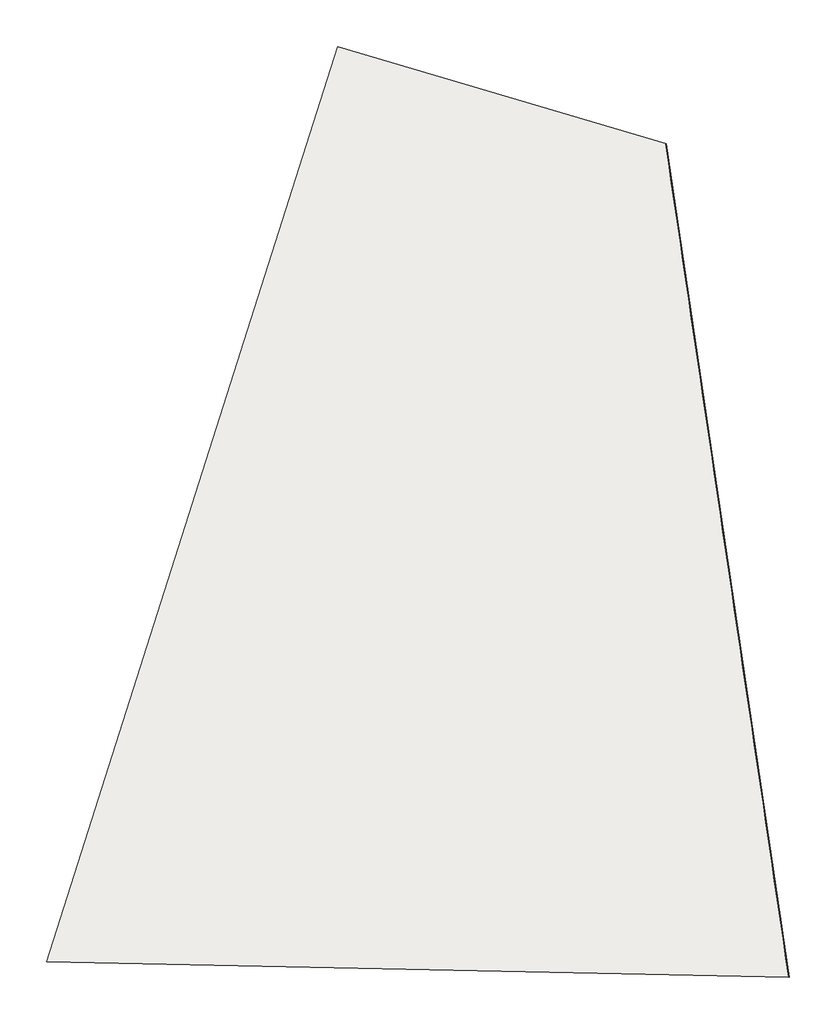
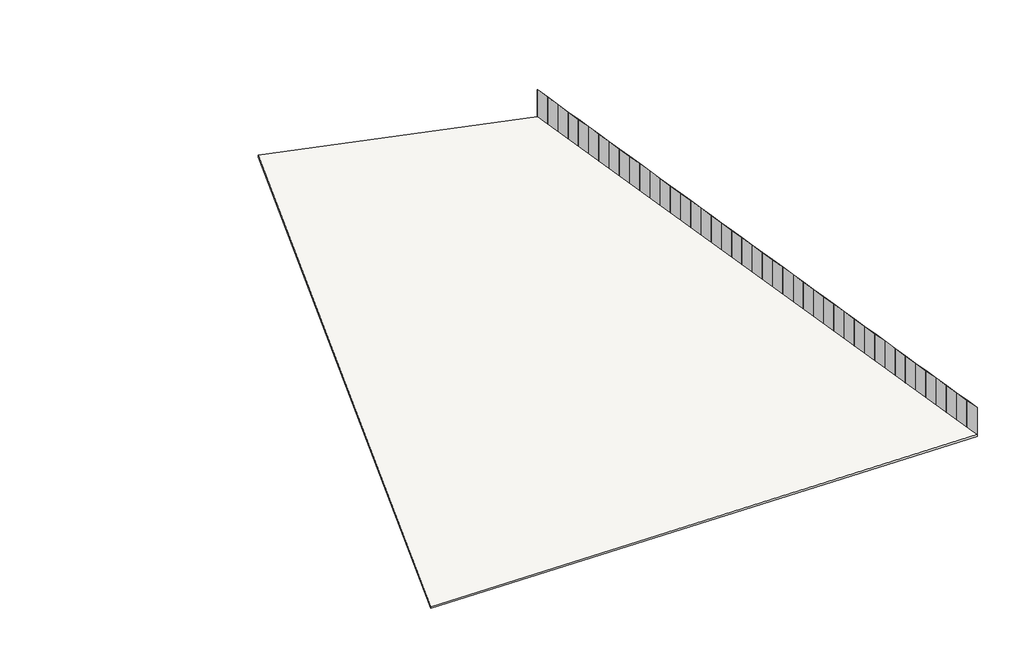
# One storey: 44 plates, 1 slab.
"""IFC4 building model written with IfcOpenShell, lengths in millimetres."""

import ifcopenshell
import ifcopenshell.guid

model = None  # the IFC model being written
_history = None  # IfcOwnerHistory: only IFC2X3 demands one
_inside = {}  # id of a spatial element -> (the spatial element, [elements in it])
_under = {}  # id of a project, library or spatial element -> (it, [spatial elements below it])
_declared = {}  # id of a project -> (the project, [libraries it declares])
_typed = {}  # id of a type object -> (the type object, [elements of that type])
_made_of = {}  # id of a material, layer set ... -> (it, [elements and type objects made of it])


def new_model(schema):
    """Start an empty IFC model of exactly this schema.

    Asked for "IFC4X3", IfcOpenShell would pick the latest addendum, in which some entities
    have other attributes; the version numbers below select the first issue.
    IFC2X3 requires an IfcOwnerHistory on every rooted entity: one is made here for all.
    """
    global model, _history
    if schema == "IFC4X3":
        model = ifcopenshell.file(schema_version=(4, 3, 0, 0))
    else:
        model = ifcopenshell.file(schema=schema)
    _inside.clear()
    _under.clear()
    _declared.clear()
    _typed.clear()
    _made_of.clear()
    _history = None
    if model.schema == "IFC2X3":
        org = make("IfcOrganization", Name="unknown")
        user = make(
            "IfcPersonAndOrganization",
            ThePerson=make("IfcPerson", FamilyName="unknown"),
            TheOrganization=org,
        )
        app = make(
            "IfcApplication",
            ApplicationDeveloper=org,
            Version="unknown",
            ApplicationFullName="unknown",
            ApplicationIdentifier="unknown",
        )
        _history = make(
            "IfcOwnerHistory",
            OwningUser=user,
            OwningApplication=app,
            ChangeAction="ADDED",
            CreationDate=0,
        )
    return model


def make(cls, **values):
    """One entity of the class cls with the attributes given. An attribute that is None is left unset."""
    return model.create_entity(
        cls, **{name: value for name, value in values.items() if value is not None}
    )


def rooted(cls, **values):
    """An entity with a GlobalId (a new one), such as an element, a storey or a relation."""
    return make(cls, GlobalId=ifcopenshell.guid.new(), OwnerHistory=_history, **values)


def si_unit(unit_type, name, prefix=None):
    """IfcSIUnit, for example si_unit("LENGTHUNIT", "METRE", prefix="MILLI")."""
    return make("IfcSIUnit", UnitType=unit_type, Prefix=prefix, Name=name)


def assignment(units):
    """IfcUnitAssignment: the units of a project."""
    return None if units is None else make("IfcUnitAssignment", Units=units)


def point(xyz):
    """IfcCartesianPoint."""
    return None if xyz is None else make("IfcCartesianPoint", Coordinates=xyz)


def direction(xyz):
    """IfcDirection."""
    return None if xyz is None else make("IfcDirection", DirectionRatios=xyz)


def frame(location, z_axis=None, x_axis=None):
    """IfcAxis2Placement3D, a coordinate frame: its origin and axes. An axis left out is left unset."""
    return make(
        "IfcAxis2Placement3D",
        Location=point(location),
        Axis=direction(z_axis),
        RefDirection=direction(x_axis),
    )


def origin():
    """The frame at (0, 0, 0) with its axes left unset."""
    return frame((0.0, 0.0, 0.0))


def origin_with_axes():
    """The frame at (0, 0, 0) with the z axis (0, 0, 1) and the x axis (1, 0, 0) written out."""
    return frame((0.0, 0.0, 0.0), z_axis=(0.0, 0.0, 1.0), x_axis=(1.0, 0.0, 0.0))


def place(relative_to, where):
    """IfcLocalPlacement: puts the frame where relative to a parent placement (None: the world)."""
    return make(
        "IfcLocalPlacement", PlacementRelTo=relative_to, RelativePlacement=where
    )


def context(
    kind, dimensions, precision=None, world=None, true_north=None, identifier=None
):
    """IfcGeometricRepresentationContext, for example the 3D "Model" context."""
    return make(
        "IfcGeometricRepresentationContext",
        ContextIdentifier=identifier,
        ContextType=kind,
        CoordinateSpaceDimension=dimensions,
        Precision=precision,
        WorldCoordinateSystem=world,
        TrueNorth=true_north,
    )


def project(units=None, contexts=None):
    """IfcProject with its units and contexts."""
    return rooted(
        "IfcProject",
        Name="project",
        RepresentationContexts=contexts,
        UnitsInContext=assignment(units),
    )


def spatial(cls, under=None, at=None, **own):
    """A site, building, storey or space (cls), placed at a placement, below another one or the project."""
    s = rooted(cls, ObjectPlacement=at, **own)
    if under is not None:
        _under.setdefault(under.id(), (under, []))[1].append(s)
    return s


def polyline(points):
    """IfcPolyline through the points."""
    return make("IfcPolyline", Points=[point(p) for p in points])


def outline(outer, holes=None, kind="AREA"):
    """IfcArbitraryClosedProfileDef: a profile drawn as a closed curve; with holes, ...WithVoids."""
    if holes is None:
        return make("IfcArbitraryClosedProfileDef", ProfileType=kind, OuterCurve=outer)
    return make(
        "IfcArbitraryProfileDefWithVoids",
        ProfileType=kind,
        OuterCurve=outer,
        InnerCurves=holes,
    )


def extrude(swept, where, along, depth):
    """IfcExtrudedAreaSolid: the profile swept, set in the frame where, extruded along a direction by depth."""
    return make(
        "IfcExtrudedAreaSolid",
        SweptArea=swept,
        Position=where,
        ExtrudedDirection=direction(along),
        Depth=depth,
    )


def shape(context_of_items, identifier, shape_type, items):
    """IfcShapeRepresentation: the items that make up one representation, for example the "Body"."""
    return make(
        "IfcShapeRepresentation",
        ContextOfItems=context_of_items,
        RepresentationIdentifier=identifier,
        RepresentationType=shape_type,
        Items=items,
    )


def source(mapping_origin, context_of_items, identifier, shape_type, items):
    """IfcRepresentationMap: a shape defined once, which mapped items show again and again."""
    return make(
        "IfcRepresentationMap",
        MappingOrigin=mapping_origin,
        MappedRepresentation=shape(context_of_items, identifier, shape_type, items),
    )


def transform(
    local_origin,
    x_axis=None,
    y_axis=None,
    z_axis=None,
    scale=None,
    scale2=None,
    scale3=None,
    uniform=True,
):
    """IfcCartesianTransformationOperator3D, or its non-uniform kind. x_axis, y_axis, z_axis: its Axis1, 2, 3."""
    if uniform:
        return make(
            "IfcCartesianTransformationOperator3D",
            Axis1=direction(x_axis),
            Axis2=direction(y_axis),
            LocalOrigin=point(local_origin),
            Scale=scale,
            Axis3=direction(z_axis),
        )
    return make(
        "IfcCartesianTransformationOperator3DnonUniform",
        Axis1=direction(x_axis),
        Axis2=direction(y_axis),
        LocalOrigin=point(local_origin),
        Scale=scale,
        Axis3=direction(z_axis),
        Scale2=scale2,
        Scale3=scale3,
    )


def mapped(mapping_source, mapping_target):
    """IfcMappedItem: shows the shape of a source again, moved by a transform."""
    return make(
        "IfcMappedItem", MappingSource=mapping_source, MappingTarget=mapping_target
    )


def made_of(thing, what):
    """Note that an element or type object is made of a material, layer set ...; save() writes the relation."""
    if what is not None:
        _made_of.setdefault(what.id(), (what, []))[1].append(thing)
    return thing


def element(
    cls,
    number,
    at=None,
    inside=None,
    cuts=None,
    type_object=None,
    material=None,
    context=None,
    identifier="Body",
    shape_type=None,
    held_by="IfcProductDefinitionShape",
    body=None,
    shapes=None,
    **own,
):
    """One element of the class cls, such as IfcWall. Its Tag is "e" and its number.

    at: its placement. inside: the storey or other place that contains it. cuts: it is an
    opening in that element (IfcRelVoidsElement). A single representation is given by context,
    identifier, shape_type and body (its items); several are given by shapes. held_by: the class
    of the entity that holds the representations. save() writes the other relations.
    """
    e = rooted(cls, Tag="e%d" % number, ObjectPlacement=at, **own)
    if body is not None:
        shapes = [shape(context, identifier, shape_type, body)]
    if shapes is not None:
        e.Representation = make(held_by, Representations=shapes)
    if inside is not None:
        _inside.setdefault(inside.id(), (inside, []))[1].append(e)
    if cuts is not None:
        rooted(
            "IfcRelVoidsElement", RelatingBuildingElement=cuts, RelatedOpeningElement=e
        )
    if type_object is not None:
        _typed.setdefault(type_object.id(), (type_object, []))[1].append(e)
    return made_of(e, material)


def aggregate(whole, parts):
    """IfcRelAggregates: a whole, such as a stair, and the parts it consists of."""
    return rooted("IfcRelAggregates", RelatingObject=whole, RelatedObjects=parts)


def save(model, path):
    """Write the relations noted so far, then the file.

    IfcRelAggregates (storeys below a building ...), IfcRelContainedInSpatialStructure (elements
    in a storey), IfcRelDefinesByType, IfcRelAssociatesMaterial and IfcRelDeclares: one each for
    every whole, place, type object, material and project.
    """
    for whole, parts in _under.values():
        aggregate(whole, parts)
    for where, things in _inside.values():
        rooted(
            "IfcRelContainedInSpatialStructure",
            RelatedElements=things,
            RelatingStructure=where,
        )
    for kind, things in _typed.values():
        rooted("IfcRelDefinesByType", RelatedObjects=things, RelatingType=kind)
    for what, things in _made_of.values():
        rooted("IfcRelAssociatesMaterial", RelatedObjects=things, RelatingMaterial=what)
    for by, libraries in _declared.values():
        rooted("IfcRelDeclares", RelatingContext=by, RelatedDefinitions=libraries)
    model.write(path)


def painel_do_sistema_1cdad03e(model_context):
    return source(origin(), model_context, "Body", "SweptSolid", [
        extrude(outline(polyline([(1500.0, 24.5), (-1500.0, 24.5), (-1500.0, 49.5), (1500.0, 49.5), (1500.0, 24.5)])), origin_with_axes(), (0.0, 0.0, 1.0), 1500.0),
    ])


def painel_do_sistema_6129cf31(model_context):
    return source(origin(), model_context, "Body", "SweptSolid", [
        extrude(outline(polyline([(0.0, -1500.0), (0.0, -332.3130513), (0.0, 1500.0), (20.0931032, 1500.0), (20.0931032, -1500.0), (0.0, -1500.0)])), frame((0.0, 24.5, 0.0), z_axis=(0.0, 1.0, 0.0), x_axis=(0.0, 0.0, 1.0)), (0.0, 0.0, 1.0), 25.0),
    ])


model = new_model("IFC4")

# Units and contexts
model_context = context("Model", 3, world=origin())
ifc_project = project(units=[si_unit("LENGTHUNIT", "METRE", prefix="MILLI")], contexts=[model_context])

# Site, building, storey
site = spatial("IfcSite", under=ifc_project)
building = spatial("IfcBuilding", under=site)
storey = spatial("IfcBuildingStorey", under=building, Name="Nível 2", Elevation=3000.0)

# Plates
placement = place(None, origin())
painel_do_sistema_shape = painel_do_sistema_1cdad03e(model_context)
element("IfcPlate", 1, ObjectType="Painel do sistema : Envidraçado", at=placement, inside=storey, context=model_context, shape_type="MappedRepresentation", body=[
    mapped(painel_do_sistema_shape, transform((27835.0106579, -36774.1442579, 4500.000015), x_axis=(0.0, 0.0, 1.0), y_axis=(-0.9892699032546328, -0.1460994815684493, 0.0), z_axis=(0.1460994815684493, -0.9892699032546328, 0.0))),
])
element("IfcPlate", 2, ObjectType="Painel do sistema : Envidraçado", at=placement, inside=storey, context=model_context, shape_type="MappedRepresentation", body=[
    mapped(painel_do_sistema_shape, transform((27615.8614356, -35290.239403, 4500.000015), x_axis=(0.0, 0.0, 1.0), y_axis=(-0.9892699032546328, -0.14609948156844887, 0.0), z_axis=(0.14609948156844887, -0.9892699032546328, 0.0))),
])
element("IfcPlate", 3, ObjectType="Painel do sistema : Envidraçado", at=placement, inside=storey, context=model_context, shape_type="MappedRepresentation", body=[
    mapped(painel_do_sistema_shape, transform((27396.7122132, -33806.3345481, 4500.000015), x_axis=(0.0, 0.0, 1.0), y_axis=(-0.9892699032546323, -0.1460994815684521, 0.0), z_axis=(0.1460994815684521, -0.9892699032546323, 0.0))),
])
element("IfcPlate", 4, ObjectType="Painel do sistema : Envidraçado", at=placement, inside=storey, context=model_context, shape_type="MappedRepresentation", body=[
    mapped(painel_do_sistema_shape, transform((27177.5629909, -32322.4296932, 4500.000015), x_axis=(0.0, 0.0, 1.0), y_axis=(-0.9892699032546327, -0.14609948156844926, 0.0), z_axis=(0.14609948156844926, -0.9892699032546327, 0.0))),
])
element("IfcPlate", 5, ObjectType="Painel do sistema : Envidraçado", at=placement, inside=storey, context=model_context, shape_type="MappedRepresentation", body=[
    mapped(painel_do_sistema_shape, transform((26958.4137685, -30838.5248383, 4500.000015), x_axis=(0.0, 0.0, 1.0), y_axis=(-0.9892699032546327, -0.1460994815684493, 0.0), z_axis=(0.1460994815684493, -0.9892699032546327, 0.0))),
])
element("IfcPlate", 6, ObjectType="Painel do sistema : Envidraçado", at=placement, inside=storey, context=model_context, shape_type="MappedRepresentation", body=[
    mapped(painel_do_sistema_shape, transform((26739.2645462, -29354.6199835, 4500.000015), x_axis=(0.0, 0.0, 1.0), y_axis=(-0.9892699032546327, -0.1460994815684493, 0.0), z_axis=(0.1460994815684493, -0.9892699032546327, 0.0))),
])
element("IfcPlate", 7, ObjectType="Painel do sistema : Envidraçado", at=placement, inside=storey, context=model_context, shape_type="MappedRepresentation", body=[
    mapped(painel_do_sistema_shape, transform((26520.1153238, -27870.7151286, 4500.000015), x_axis=(0.0, 0.0, 1.0), y_axis=(-0.9892699032546324, -0.1460994815684517, 0.0), z_axis=(0.1460994815684517, -0.9892699032546324, 0.0))),
])
element("IfcPlate", 8, ObjectType="Painel do sistema : Envidraçado", at=placement, inside=storey, context=model_context, shape_type="MappedRepresentation", body=[
    mapped(painel_do_sistema_shape, transform((26300.9661014, -26386.8102737, 4500.000015), x_axis=(0.0, 0.0, 1.0), y_axis=(-0.9892699032546328, -0.1460994815684493, 0.0), z_axis=(0.1460994815684493, -0.9892699032546328, 0.0))),
])
element("IfcPlate", 9, ObjectType="Painel do sistema : Envidraçado", at=placement, inside=storey, context=model_context, shape_type="MappedRepresentation", body=[
    mapped(painel_do_sistema_shape, transform((26081.8168791, -24902.9054188, 4500.000015), x_axis=(0.0, 0.0, 1.0), y_axis=(-0.9892699032546328, -0.14609948156844887, 0.0), z_axis=(0.14609948156844887, -0.9892699032546328, 0.0))),
])
element("IfcPlate", 10, ObjectType="Painel do sistema : Envidraçado", at=placement, inside=storey, context=model_context, shape_type="MappedRepresentation", body=[
    mapped(painel_do_sistema_shape, transform((25862.6676567, -23419.0005639, 4500.000015), x_axis=(0.0, 0.0, 1.0), y_axis=(-0.9892699032546324, -0.1460994815684517, 0.0), z_axis=(0.1460994815684517, -0.9892699032546324, 0.0))),
])
element("IfcPlate", 11, ObjectType="Painel do sistema : Envidraçado", at=placement, inside=storey, context=model_context, shape_type="MappedRepresentation", body=[
    mapped(painel_do_sistema_shape, transform((25643.5184344, -21935.095709, 4500.000015), x_axis=(0.0, 0.0, 1.0), y_axis=(-0.9892699032546328, -0.1460994815684493, 0.0), z_axis=(0.1460994815684493, -0.9892699032546328, 0.0))),
])
element("IfcPlate", 12, ObjectType="Painel do sistema : Envidraçado", at=placement, inside=storey, context=model_context, shape_type="MappedRepresentation", body=[
    mapped(painel_do_sistema_shape, transform((25424.369212, -20451.1908542, 4500.000015), x_axis=(0.0, 0.0, 1.0), y_axis=(-0.9892699032546324, -0.1460994815684517, 0.0), z_axis=(0.1460994815684517, -0.9892699032546324, 0.0))),
])
element("IfcPlate", 13, ObjectType="Painel do sistema : Envidraçado", at=placement, inside=storey, context=model_context, shape_type="MappedRepresentation", body=[
    mapped(painel_do_sistema_shape, transform((25205.2199897, -18967.2859993, 4500.000015), x_axis=(0.0, 0.0, 1.0), y_axis=(-0.9892699032546328, -0.14609948156844868, 0.0), z_axis=(0.14609948156844868, -0.9892699032546328, 0.0))),
])
element("IfcPlate", 14, ObjectType="Painel do sistema : Envidraçado", at=placement, inside=storey, context=model_context, shape_type="MappedRepresentation", body=[
    mapped(painel_do_sistema_shape, transform((24986.0707673, -17483.3811444, 4500.000015), x_axis=(0.0, 0.0, 1.0), y_axis=(-0.9892699032546328, -0.1460994815684491, 0.0), z_axis=(0.1460994815684491, -0.9892699032546328, 0.0))),
])
element("IfcPlate", 15, ObjectType="Painel do sistema : Envidraçado", at=placement, inside=storey, context=model_context, shape_type="MappedRepresentation", body=[
    mapped(painel_do_sistema_shape, transform((24766.921545, -15999.4762895, 4500.000015), x_axis=(0.0, 0.0, 1.0), y_axis=(-0.9892699032546328, -0.1460994815684493, 0.0), z_axis=(0.1460994815684493, -0.9892699032546328, 0.0))),
])
element("IfcPlate", 16, ObjectType="Painel do sistema : Envidraçado", at=placement, inside=storey, context=model_context, shape_type="MappedRepresentation", body=[
    mapped(painel_do_sistema_shape, transform((24547.7723226, -14515.5714346, 4500.000015), x_axis=(0.0, 0.0, 1.0), y_axis=(-0.9892699032546324, -0.1460994815684517, 0.0), z_axis=(0.1460994815684517, -0.9892699032546324, 0.0))),
])
element("IfcPlate", 17, ObjectType="Painel do sistema : Envidraçado", at=placement, inside=storey, context=model_context, shape_type="MappedRepresentation", body=[
    mapped(painel_do_sistema_shape, transform((24328.6231003, -13031.6665798, 4500.000015), x_axis=(0.0, 0.0, 1.0), y_axis=(-0.9892699032546327, -0.1460994815684495, 0.0), z_axis=(0.1460994815684495, -0.9892699032546327, 0.0))),
])
element("IfcPlate", 18, ObjectType="Painel do sistema : Envidraçado", at=placement, inside=storey, context=model_context, shape_type="MappedRepresentation", body=[
    mapped(painel_do_sistema_shape, transform((24109.4738779, -11547.7617249, 4500.000015), x_axis=(0.0, 0.0, 1.0), y_axis=(-0.9892699032546328, -0.1460994815684491, 0.0), z_axis=(0.1460994815684491, -0.9892699032546328, 0.0))),
])
element("IfcPlate", 19, ObjectType="Painel do sistema : Envidraçado", at=placement, inside=storey, context=model_context, shape_type="MappedRepresentation", body=[
    mapped(painel_do_sistema_shape, transform((23890.3246556, -10063.85687, 4500.000015), x_axis=(0.0, 0.0, 1.0), y_axis=(-0.9892699032546324, -0.14609948156845148, 0.0), z_axis=(0.14609948156845148, -0.9892699032546324, 0.0))),
])
element("IfcPlate", 20, ObjectType="Painel do sistema : Envidraçado", at=placement, inside=storey, context=model_context, shape_type="MappedRepresentation", body=[
    mapped(painel_do_sistema_shape, transform((23671.1754332, -8579.9520151, 4500.000015), x_axis=(0.0, 0.0, 1.0), y_axis=(-0.9892699032546332, -0.14609948156844624, 0.0), z_axis=(0.14609948156844624, -0.9892699032546332, 0.0))),
])
element("IfcPlate", 21, ObjectType="Painel do sistema : Envidraçado", at=placement, inside=storey, context=model_context, shape_type="MappedRepresentation", body=[
    mapped(painel_do_sistema_shape, transform((23452.0262109, -7096.0471602, 4500.000015), x_axis=(0.0, 0.0, 1.0), y_axis=(-0.9892699032546319, -0.14609948156845473, 0.0), z_axis=(0.14609948156845473, -0.9892699032546319, 0.0))),
])
element("IfcPlate", 22, ObjectType="Painel do sistema : Envidraçado", at=placement, inside=storey, context=model_context, shape_type="MappedRepresentation", body=[
    mapped(painel_do_sistema_shape, transform((23232.8769885, -5612.1423053, 4500.000015), x_axis=(0.0, 0.0, 1.0), y_axis=(-0.9892699032546332, -0.14609948156844646, 0.0), z_axis=(0.14609948156844646, -0.9892699032546332, 0.0))),
])
element("IfcPlate", 23, ObjectType="Painel do sistema : Envidraçado", at=placement, inside=storey, context=model_context, shape_type="MappedRepresentation", body=[
    mapped(painel_do_sistema_shape, transform((23013.7277662, -4128.2374505, 4500.000015), x_axis=(0.0, 0.0, 1.0), y_axis=(-0.9892699032546324, -0.1460994815684517, 0.0), z_axis=(0.1460994815684517, -0.9892699032546324, 0.0))),
])
element("IfcPlate", 24, ObjectType="Painel do sistema : Envidraçado", at=placement, inside=storey, context=model_context, shape_type="MappedRepresentation", body=[
    mapped(painel_do_sistema_shape, transform((22794.5785438, -2644.3325956, 4500.000015), x_axis=(0.0, 0.0, 1.0), y_axis=(-0.9892699032546328, -0.14609948156844865, 0.0), z_axis=(0.14609948156844865, -0.9892699032546328, 0.0))),
])
element("IfcPlate", 25, ObjectType="Painel do sistema : Envidraçado", at=placement, inside=storey, context=model_context, shape_type="MappedRepresentation", body=[
    mapped(painel_do_sistema_shape, transform((22575.4293215, -1160.4277407, 4500.000015), x_axis=(0.0, 0.0, 1.0), y_axis=(-0.9892699032546327, -0.1460994815684493, 0.0), z_axis=(0.1460994815684493, -0.9892699032546327, 0.0))),
])
element("IfcPlate", 26, ObjectType="Painel do sistema : Envidraçado", at=placement, inside=storey, context=model_context, shape_type="MappedRepresentation", body=[
    mapped(painel_do_sistema_shape, transform((22356.2800991, 323.4771142, 4500.000015), x_axis=(0.0, 0.0, 1.0), y_axis=(-0.9892699032546324, -0.14609948156845148, 0.0), z_axis=(0.14609948156845148, -0.9892699032546324, 0.0))),
])
element("IfcPlate", 27, ObjectType="Painel do sistema : Envidraçado", at=placement, inside=storey, context=model_context, shape_type="MappedRepresentation", body=[
    mapped(painel_do_sistema_shape, transform((22137.1308767, 1807.3819691, 4500.000015), x_axis=(0.0, 0.0, 1.0), y_axis=(-0.9892699032546332, -0.1460994815684469, 0.0), z_axis=(0.1460994815684469, -0.9892699032546332, 0.0))),
])
element("IfcPlate", 28, ObjectType="Painel do sistema : Envidraçado", at=placement, inside=storey, context=model_context, shape_type="MappedRepresentation", body=[
    mapped(painel_do_sistema_shape, transform((21917.9816544, 3291.2868239, 4500.000015), x_axis=(0.0, 0.0, 1.0), y_axis=(-0.9892699032546323, -0.1460994815684521, 0.0), z_axis=(0.1460994815684521, -0.9892699032546323, 0.0))),
])
element("IfcPlate", 29, ObjectType="Painel do sistema : Envidraçado", at=placement, inside=storey, context=model_context, shape_type="MappedRepresentation", body=[
    mapped(painel_do_sistema_shape, transform((21698.832432, 4775.1916788, 4500.000015), x_axis=(0.0, 0.0, 1.0), y_axis=(-0.9892699032546323, -0.14609948156845232, 0.0), z_axis=(0.14609948156845232, -0.9892699032546323, 0.0))),
])
element("IfcPlate", 30, ObjectType="Painel do sistema : Envidraçado", at=placement, inside=storey, context=model_context, shape_type="MappedRepresentation", body=[
    mapped(painel_do_sistema_shape, transform((21479.6832097, 6259.0965337, 4500.000015), x_axis=(0.0, 0.0, 1.0), y_axis=(-0.9892699032546332, -0.14609948156844646, 0.0), z_axis=(0.14609948156844646, -0.9892699032546332, 0.0))),
])
element("IfcPlate", 31, ObjectType="Painel do sistema : Envidraçado", at=placement, inside=storey, context=model_context, shape_type="MappedRepresentation", body=[
    mapped(painel_do_sistema_shape, transform((21260.5339873, 7743.0013886, 4500.000015), x_axis=(0.0, 0.0, 1.0), y_axis=(-0.9892699032546323, -0.14609948156845232, 0.0), z_axis=(0.14609948156845232, -0.9892699032546323, 0.0))),
])
element("IfcPlate", 32, ObjectType="Painel do sistema : Envidraçado", at=placement, inside=storey, context=model_context, shape_type="MappedRepresentation", body=[
    mapped(painel_do_sistema_shape, transform((21041.384765, 9226.9062435, 4500.000015), x_axis=(0.0, 0.0, 1.0), y_axis=(-0.9892699032546327, -0.1460994815684495, 0.0), z_axis=(0.1460994815684495, -0.9892699032546327, 0.0))),
])
element("IfcPlate", 33, ObjectType="Painel do sistema : Envidraçado", at=placement, inside=storey, context=model_context, shape_type="MappedRepresentation", body=[
    mapped(painel_do_sistema_shape, transform((20822.2355426, 10710.8110984, 4500.000015), x_axis=(0.0, 0.0, 1.0), y_axis=(-0.9892699032546327, -0.1460994815684495, 0.0), z_axis=(0.1460994815684495, -0.9892699032546327, 0.0))),
])
element("IfcPlate", 34, ObjectType="Painel do sistema : Envidraçado", at=placement, inside=storey, context=model_context, shape_type="MappedRepresentation", body=[
    mapped(painel_do_sistema_shape, transform((20603.0863203, 12194.7159532, 4500.000015), x_axis=(0.0, 0.0, 1.0), y_axis=(-0.9892699032546327, -0.1460994815684495, 0.0), z_axis=(0.1460994815684495, -0.9892699032546327, 0.0))),
])
element("IfcPlate", 35, ObjectType="Painel do sistema : Envidraçado", at=placement, inside=storey, context=model_context, shape_type="MappedRepresentation", body=[
    mapped(painel_do_sistema_shape, transform((20383.9370979, 13678.6208081, 4500.000015), x_axis=(0.0, 0.0, 1.0), y_axis=(-0.9892699032546326, -0.14609948156845054, 0.0), z_axis=(0.14609948156845054, -0.9892699032546326, 0.0))),
])
element("IfcPlate", 36, ObjectType="Painel do sistema : Envidraçado", at=placement, inside=storey, context=model_context, shape_type="MappedRepresentation", body=[
    mapped(painel_do_sistema_shape, transform((20164.7878756, 15162.525663, 4500.000015), x_axis=(0.0, 0.0, 1.0), y_axis=(-0.9892699032546328, -0.14609948156844887, 0.0), z_axis=(0.14609948156844887, -0.9892699032546328, 0.0))),
])
element("IfcPlate", 37, ObjectType="Painel do sistema : Envidraçado", at=placement, inside=storey, context=model_context, shape_type="MappedRepresentation", body=[
    mapped(painel_do_sistema_shape, transform((19945.6386532, 16646.4305179, 4500.000015), x_axis=(0.0, 0.0, 1.0), y_axis=(-0.9892699032546327, -0.1460994815684493, 0.0), z_axis=(0.1460994815684493, -0.9892699032546327, 0.0))),
])
element("IfcPlate", 38, ObjectType="Painel do sistema : Envidraçado", at=placement, inside=storey, context=model_context, shape_type="MappedRepresentation", body=[
    mapped(painel_do_sistema_shape, transform((19726.4894309, 18130.3353728, 4500.000015), x_axis=(0.0, 0.0, 1.0), y_axis=(-0.9892699032546326, -0.14609948156845012, 0.0), z_axis=(0.14609948156845012, -0.9892699032546326, 0.0))),
])
element("IfcPlate", 39, ObjectType="Painel do sistema : Envidraçado", at=placement, inside=storey, context=model_context, shape_type="MappedRepresentation", body=[
    mapped(painel_do_sistema_shape, transform((19507.3402085, 19614.2402276, 4500.000015), x_axis=(0.0, 0.0, 1.0), y_axis=(-0.9892699032546329, -0.14609948156844846, 0.0), z_axis=(0.14609948156844846, -0.9892699032546329, 0.0))),
])
element("IfcPlate", 40, ObjectType="Painel do sistema : Envidraçado", at=placement, inside=storey, context=model_context, shape_type="MappedRepresentation", body=[
    mapped(painel_do_sistema_shape, transform((19288.1909862, 21098.1450825, 4500.000015), x_axis=(0.0, 0.0, 1.0), y_axis=(-0.9892699032546323, -0.14609948156845254, 0.0), z_axis=(0.14609948156845254, -0.9892699032546323, 0.0))),
])
element("IfcPlate", 41, ObjectType="Painel do sistema : Envidraçado", at=placement, inside=storey, context=model_context, shape_type="MappedRepresentation", body=[
    mapped(painel_do_sistema_shape, transform((19069.0417638, 22582.0499374, 4500.000015), x_axis=(0.0, 0.0, 1.0), y_axis=(-0.9892699032546326, -0.1460994815684497, 0.0), z_axis=(0.1460994815684497, -0.9892699032546326, 0.0))),
])
element("IfcPlate", 42, ObjectType="Painel do sistema : Envidraçado", at=placement, inside=storey, context=model_context, shape_type="MappedRepresentation", body=[
    mapped(painel_do_sistema_shape, transform((18849.8925415, 24065.9547923, 4500.000015), x_axis=(0.0, 0.0, 1.0), y_axis=(-0.9892699032546326, -0.14609948156845012, 0.0), z_axis=(0.14609948156845012, -0.9892699032546326, 0.0))),
])
element("IfcPlate", 43, ObjectType="Painel do sistema : Envidraçado", at=placement, inside=storey, context=model_context, shape_type="MappedRepresentation", body=[
    mapped(painel_do_sistema_shape, transform((18630.7433191, 25549.8596472, 4500.000015), x_axis=(0.0, 0.0, 1.0), y_axis=(-0.9892699032546326, -0.14609948156844982, 0.0), z_axis=(0.14609948156844982, -0.9892699032546326, 0.0))),
])
painel_do_sistema_2_shape = painel_do_sistema_6129cf31(model_context)
element("IfcPlate", 44, ObjectType="Painel do sistema : Envidraçado", at=placement, inside=storey, context=model_context, shape_type="MappedRepresentation", body=[
    mapped(painel_do_sistema_2_shape, transform((18627.8077271, 25569.7371494, 4500.000015), x_axis=(0.0, 0.0, 1.0), y_axis=(-0.9892699032546369, -0.14609948156842112, 0.0), z_axis=(0.14609948156842112, -0.9892699032546369, 0.0))),
])

# Slab
element("IfcSlab", 45, ObjectType="piso aula 04", at=placement, inside=storey, context=model_context, shape_type="SweptSolid", body=[
    extrude(outline(polyline([(-6526.0277886, 32996.9225357), (18627.8077271, 25569.7371494), (28054.1598803, -38258.0491127), (-28815.2621129, -37063.5346132), (-6526.0277886, 32996.9225357)])), frame((0.0, 0.0, 2790.0), z_axis=(0.0, 0.0, 1.0), x_axis=(1.0, 0.0, 0.0)), (0.0, 0.0, 1.0), 210.0),
])

save(model, "model.ifc")

# Revit data of these elements
# Project information
#   Data de emissão do projeto = "Data de emissão"
#   Status do projeto = "Status do projeto"
#   Nome do cliente = "Proprietário"
#   Endereço do projeto = "Enter address here"
#   Nome do projeto = "Nome do projeto"
#   Número do projeto = "0001"
# Type "Painel do sistema : Envidraçado"
#   Construction Type Id = "GSP4R"
#   Analytic Construction = "Vidraça única Pilkington 1/8 pol"
#   Visual Light Transmittance = 0.9
#   Solar Heat Gain Coefficient = 0.86
#   Heat Transfer Coefficient (U) = 6.7069 W/(m²·K)
# Type "piso aula 04"
#   Function = 0
#   Layers, outside or top first: 0.02 m "Azulejo cerâmico" (function 4); 0.04 m "Concreto, Faixa de areia/cimento" (function 2); 0.15 m "Concreto,  Moldado in loco" (function 1)
# Elements 1, 2, 3, 4, 5, 6, 7, 8, 9, 10, 11, 12, 13, 14, 15, 16, 17, 18, 19, 20, 21, 22, 23, 24, 25, 26, 27, 28, 29, 30, 31, 32, 33, 34, 35, 36, 37, 38, 39, 40, 41, 42, 43, 44 (IfcPlate, "Painel do sistema : Envidraçado")
#   Phase Created = Construção nova
#   Materials on its faces: "Vidro"
# Element 45 (IfcSlab, "piso aula 04")
#   built-in parameter 1001955 = 1.26278 (stored number, unit not read)
#   Height Offset From Level = 0.00 m
#   Phase Created = Construção nova
#   Materials on its faces: "Concreto,  Moldado in loco", "Azulejo cerâmico"
# Materials
#   "Azulejo cerâmico": class "Cerâmica", colour RGB 246 230 196, transparency 0, Description = "Material físico", Cost = 0
#   "Concreto, Faixa de areia/cimento": class "Concreto", colour RGB 127 127 127, transparency 0, Description = "Revestimento de laje de concreto", Cost = 0
#   "Concreto,  Moldado in loco": class "Concreto", colour RGB 192 192 192, transparency 0, Description = "Material físico", Cost = 0
#   "Vidro": class "Vidro", colour RGB 0 128 192, transparency 0.9, Description = "Vidro de sílica", Cost = 0
